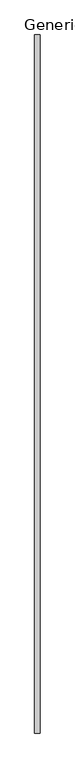
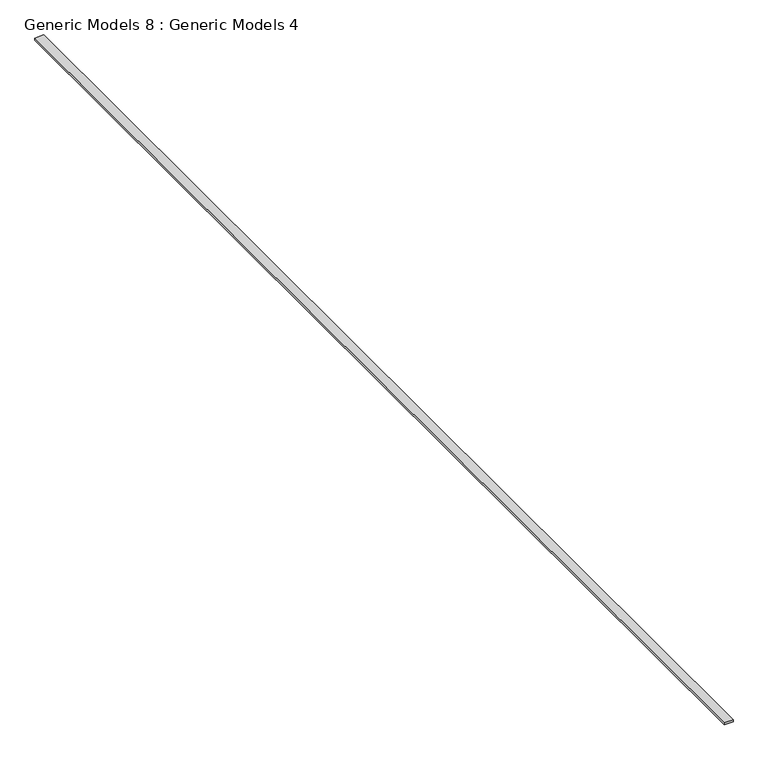
"""IFC4 building model written with IfcOpenShell, lengths in millimetres: proxy geometry, Generic Models 8 : Generic Models 4."""

from ifc_helpers import new_model, si_unit, frame, origin, place, context, project, spatial, polyline, outline, extrude, source, transform, mapped, element, save


def generic_models_8_generic_models_4_f6e08eeb(model_context):
    return source(origin(), model_context, "Body", "SweptSolid", [
        extrude(outline(polyline([(127066.3735933, 8575.5013705), (127104.4735933, 8575.5013705), (127098.6527599, 8435.8013705), (127066.3735933, 8435.8013705), (127066.3735933, 8575.5013705)])), frame((0.0, -6864.9230338, 0.0), z_axis=(0.0, 1.0, 0.0), x_axis=(0.0, 0.0, 1.0)), (0.0, 0.0, 1.0), 18643.6),
    ])


if __name__ == "__main__":
    model = new_model("IFC4")
    model_context = context("Model", 3, world=origin())
    ifc_project = project(units=[si_unit("LENGTHUNIT", "METRE", prefix="MILLI")], contexts=[model_context])
    site = spatial("IfcSite", under=ifc_project)
    building = spatial("IfcBuilding", under=site)
    placement = place(None, origin())
    generic_models_8_generic_models_4_shape = generic_models_8_generic_models_4_f6e08eeb(model_context)
    element("IfcBuildingElementProxy", 1, Name="Generic Models 8 : Generic Models 4", ObjectType="Generic Models 8 : Generic Models 4", at=placement, inside=building, context=model_context, shape_type="MappedRepresentation", body=[
        mapped(generic_models_8_generic_models_4_shape, transform((0.0, 0.0, 0.0), x_axis=(1.0, 0.0, 0.0), y_axis=(0.0, 1.0, 0.0), z_axis=(0.0, 0.0, 1.0))),
    ])
    save(model, "model.ifc")

# Revit data of these elements
# Element 1 (IfcBuildingElementProxy, "Generic Models 8 : Generic Models 4")
#   Materials on its faces: "_2X BLOCKING AS REQUIRED"
# Materials
#   "_2X BLOCKING AS REQUIRED": class "Generic", colour RGB 177 130 114, transparency 0, Cost = 0
